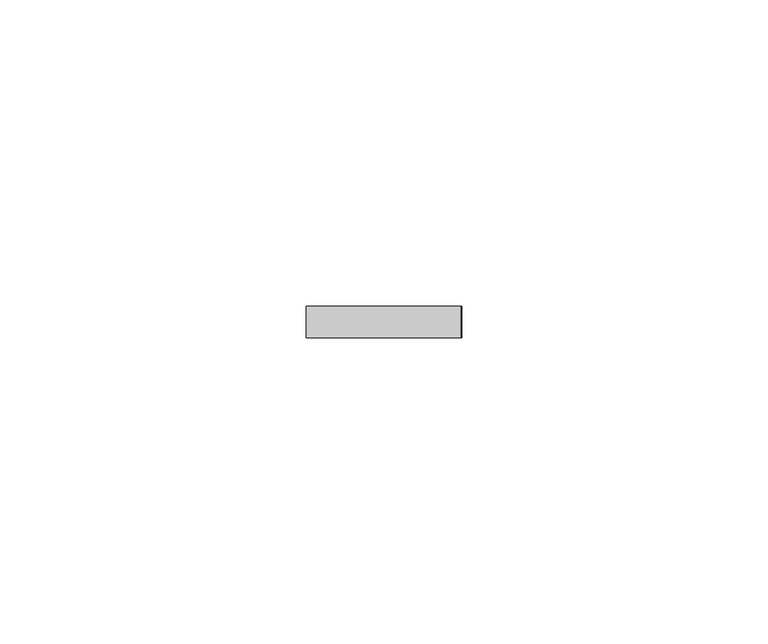
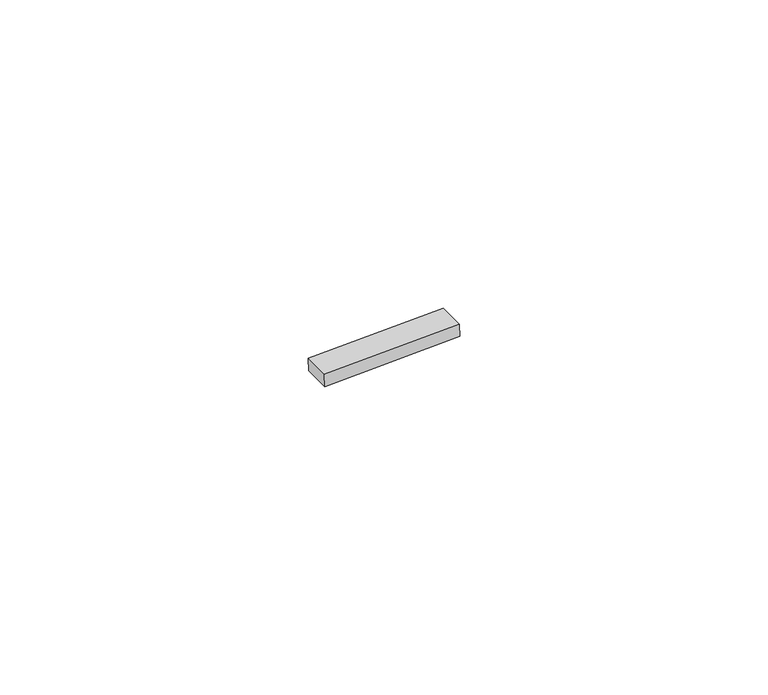
"""IFC4 building model written with IfcOpenShell, lengths in millimetres: proxy geometry, Inner panel:Inner panel:1:Inner panel:1 : Inner panel:Inner panel:300324:2:Inner panel:1:Inner panel:1 : Inner panel:Inner panel:300324:2 : Inner panel:Inner panel:1:Inner panel:1 : Inner panel:Inner panel:300324:300043:174 : Inner panel:Inner panel:1:Inner panel:1 : Inner panel:Inner panel:300324:2:Inner panel:1:Inner panel:1 : Inner panel:Inner panel:300324:2 : Inner panel:Inner panel:1:Inner panel:1 : Inner panel:Inner panel:300324:300043:308120."""

from ifc_helpers import new_model, si_unit, frame, origin, place, context, project, spatial, polyline, outline, extrude, source, transform, mapped, element, save


def generic_models_ec3ecef0(model_context):
    return source(origin(), model_context, "Body", "SweptSolid", [
        extrude(outline(polyline([(0.0, -25.4), (0.0, 0.0), (5.213809, 0.0), (5.213809, -25.4), (0.0, -25.4)])), frame((560380.9331581, -565806.907991, 3950.5346612), z_axis=(-0.041630544712223896, 0.0, 0.9991330730923502), x_axis=(0.0, -1.0, 0.0)), (0.0, 0.0, 1.0), 2.4763745),
    ])


if __name__ == "__main__":
    model = new_model("IFC4")
    model_context = context("Model", 3, world=origin())
    ifc_project = project(units=[si_unit("LENGTHUNIT", "METRE", prefix="MILLI")], contexts=[model_context])
    site = spatial("IfcSite", under=ifc_project)
    building = spatial("IfcBuilding", under=site)
    placement = place(None, origin())
    generic_models_shape = generic_models_ec3ecef0(model_context)
    element("IfcBuildingElementProxy", 1, Name="Inner panel:Inner panel:1:Inner panel:1 : Inner panel:Inner panel:300324:2:Inner panel:1:Inner panel:1 : Inner panel:Inner panel:300324:2 : Inner panel:Inner panel:1:Inner panel:1 : Inner panel:Inner panel:300324:300043:174 : Inner panel:Inner panel:1:Inner panel:1 : Inner panel:Inner panel:300324:2:Inner panel:1:Inner panel:1 : Inner panel:Inner panel:300324:2 : Inner panel:Inner panel:1:Inner panel:1 : Inner panel:Inner panel:300324:300043:308120", ObjectType="Inner panel:Inner panel:1:Inner panel:1 : Inner panel:Inner panel:300324:2:Inner panel:1:Inner panel:1 : Inner panel:Inner panel:300324:2 : Inner panel:Inner panel:1:Inner panel:1 : Inner panel:Inner panel:300324:300043:174 : Inner panel:Inner panel:1:Inner panel:1 : Inner panel:Inner panel:300324:2:Inner panel:1:Inner panel:1 : Inner panel:Inner panel:300324:2 : Inner panel:Inner panel:1:Inner panel:1 : Inner panel:Inner panel:300324:300043:308120", at=placement, inside=building, context=model_context, shape_type="MappedRepresentation", body=[
        mapped(generic_models_shape, transform((0.0, 0.0, 0.0), x_axis=(1.0, 0.0, 0.0), y_axis=(0.0, 1.0, 0.0), z_axis=(0.0, 0.0, 1.0))),
    ])
    save(model, "model.ifc")

# Revit data of these elements
# Type "Inner panel:Inner panel:1:Inner panel:1 : Inner panel:Inner panel:300324:2:Inner panel:1:Inner panel:1 : Inner panel:Inner panel:300324:2 : Inner panel:Inner panel:1:Inner panel:1 : Inner panel:Inner panel:300324:300043:174 : Inner panel:Inner panel:1:Inner panel:1 : Inner panel:Inner panel:300324:2:Inner panel:1:Inner panel:1 : Inner panel:Inner panel:300324:2 : Inner panel:Inner panel:1:Inner panel:1 : Inner panel:Inner panel:300324:300043:308120"
#   NameOverride = "Inner panel:Inner panel:1:Inner panel:1 : Inner panel:Inner panel:300324:2:Inner panel:1:Inner panel:1 : Inner panel:Inner panel:300324:2 : Inner panel:Inner panel:1:Inner panel:1 : Inner panel:Inner panel:300324:300043:308120"
#   ObjectTypeOverride = "Inner panel:1:Inner panel:1 : Inner panel:Inner panel:300324:2 : Inner panel:Inner panel:1:Inner panel:1 : Inner panel:Inner panel:300324:300043"
#   Reference = "Inner panel"
#   Tag = "308120"
# Element 1 (IfcBuildingElementProxy, "Inner panel:Inner panel:1:Inner panel:1 : Inner panel:Inner panel:300324:2:Inner panel:1:Inner panel:1 : Inner panel:Inner panel:300324:2 : Inner panel:Inner panel:1:Inner panel:1 : Inner panel:Inner panel:300324:300043:174 : Inner panel:Inner panel:1:Inner panel:1 : Inner panel:Inner panel:300324:2:Inner panel:1:Inner panel:1 : Inner panel:Inner panel:300324:2 : Inner panel:Inner panel:1:Inner panel:1 : Inner panel:Inner panel:300324:300043:308120")
#   Materials on its faces: "AT CLIP - 1\" WIDE NON ABSORBENT, WEATHER-RESISTANT NEOPRENE/EPDM/SBR FOAM"
# Materials
#   "AT CLIP - 1\" WIDE NON ABSORBENT, WEATHER-RESISTANT NEOPRENE/EPDM/SBR FOAM": class "Generic", colour RGB 85 85 85, transparency 0, Cost = 0
